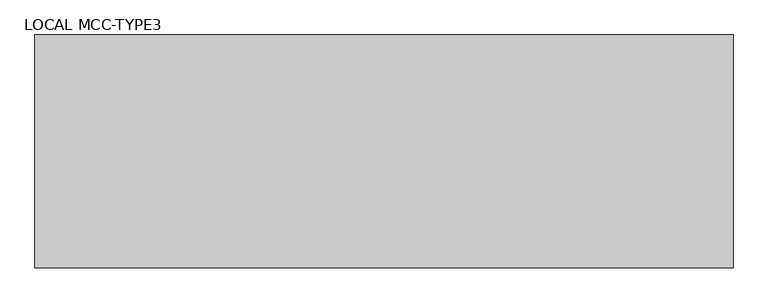
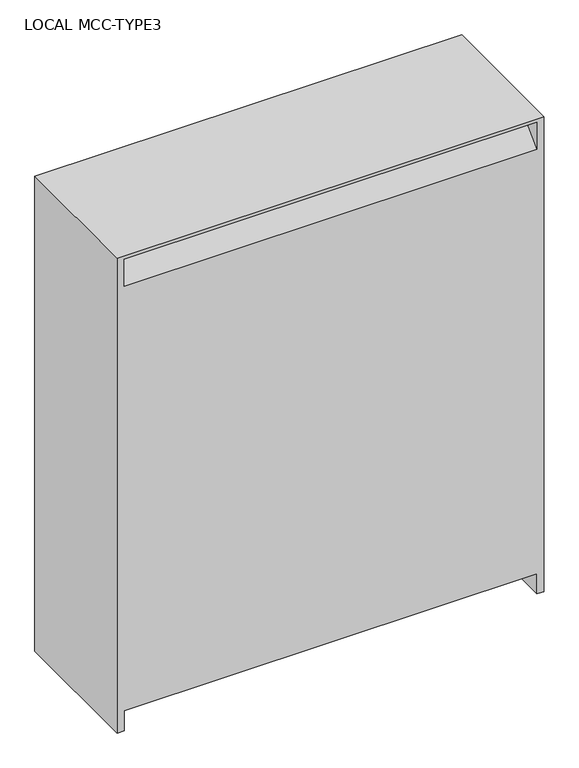
"""IFC4 building model written with IfcOpenShell, lengths in millimetres: proxy geometry, Dry Type Transformer - 480-208Y120 - NEMA Type 2 : LOCAL MCC-TYPE3."""

from ifc_helpers import new_model, si_unit, origin, place, context, project, spatial, faceted_brep, source, transform, mapped, element, save


def local_mcc_type3_fac40ae7(model_context):
    return source(origin(), model_context, "Body", "Brep", [
        faceted_brep([(762.0, -123.2841349, 1791.0), (762.0, 384.7158651, 1791.0), (-762.0, 384.7158651, 1791.0), (-762.0, -123.2841349, 1791.0), (-762.0, -123.2841349, 0.0), (-762.0, 384.7158651, 0.0), (-736.6, 384.7158651, 0.0), (-736.6, -123.2841349, 0.0), (762.0, 384.7158651, 0.0), (762.0, -123.2841349, 0.0), (736.6, -123.2841349, 0.0), (736.6, 384.7158651, 0.0), (736.6, 384.7158651, 76.2), (-736.6, 384.7158651, 76.2), (736.6, 384.7158651, 1676.7), (736.6, 384.7158651, 1778.3), (-736.6, 384.7158651, 1778.3), (-736.6, 384.7158651, 1676.7), (-736.6, -123.2841349, 76.2), (736.6, -123.2841349, 76.2), (736.6, -123.2841349, 1778.3), (736.6, -123.2841349, 1676.7), (-736.6, -123.2841349, 1676.7), (-736.6, -123.2841349, 1778.3), (736.6, -21.6841349, 1778.3), (-736.6, -21.6841349, 1778.3), (736.6, 283.1158651, 1778.3), (-736.6, 283.1158651, 1778.3)], [[[0, 1, 2, 3]], [[4, 5, 6, 7]], [[8, 9, 10, 11]], [[1, 0, 9, 8]], [[2, 1, 8, 11, 12, 13, 6, 5], [14, 15, 16, 17]], [[3, 2, 5, 4]], [[0, 3, 4, 7, 18, 19, 10, 9], [20, 21, 22, 23]], [[18, 13, 12, 19]], [[13, 18, 7, 6]], [[19, 12, 11, 10]], [[24, 21, 20]], [[25, 23, 22]], [[24, 20, 23, 25]], [[21, 24, 25, 22]], [[26, 15, 14]], [[27, 17, 16]], [[26, 14, 17, 27]], [[15, 26, 27, 16]]]),
    ])


if __name__ == "__main__":
    model = new_model("IFC4")
    model_context = context("Model", 3, world=origin())
    ifc_project = project(units=[si_unit("LENGTHUNIT", "METRE", prefix="MILLI")], contexts=[model_context])
    site = spatial("IfcSite", under=ifc_project)
    building = spatial("IfcBuilding", under=site)
    placement = place(None, origin())
    local_mcc_type3_shape = local_mcc_type3_fac40ae7(model_context)
    element("IfcBuildingElementProxy", 1, Name="Dry Type Transformer - 480-208Y120 - NEMA Type 2 : LOCAL MCC-TYPE3", ObjectType="Dry Type Transformer - 480-208Y120 - NEMA Type 2 : LOCAL MCC-TYPE3", at=placement, inside=building, context=model_context, shape_type="MappedRepresentation", body=[
        mapped(local_mcc_type3_shape, transform((0.0, 0.0, 0.0), x_axis=(1.0, 0.0, 0.0), y_axis=(0.0, 1.0, 0.0), z_axis=(0.0, 0.0, 1.0))),
    ])
    save(model, "model.ifc")

# Revit data of these elements
# Type "Dry Type Transformer - 480-208Y120 - NEMA Type 2 : LOCAL MCC-TYPE3"
#   built-in parameter 1140083 [instance default] = "Type 2"
#   Transformer Length = 1524 mm
#   Primary Voltage = 480 V
#   Transformer Height = 1791 mm
#   built-in parameter 1140140 [instance default] = 1 (stored number, unit not read)
#   Transformer Width = 508 mm
#   built-in parameter 1140142 [instance default] = -1
#   Primary Number of Poles = 3
#   built-in parameter 1140079 [instance default] = 3
#   Transformer Material = none
#   Load Classification = Transformer
#   Default Elevation = 0
#   Assembly Code = ""
#   built-in parameter 1140087 [instance default] = 1
